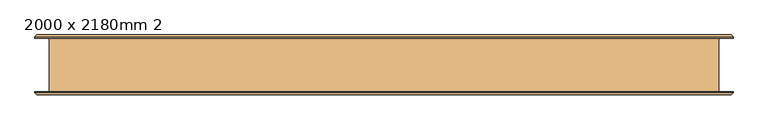
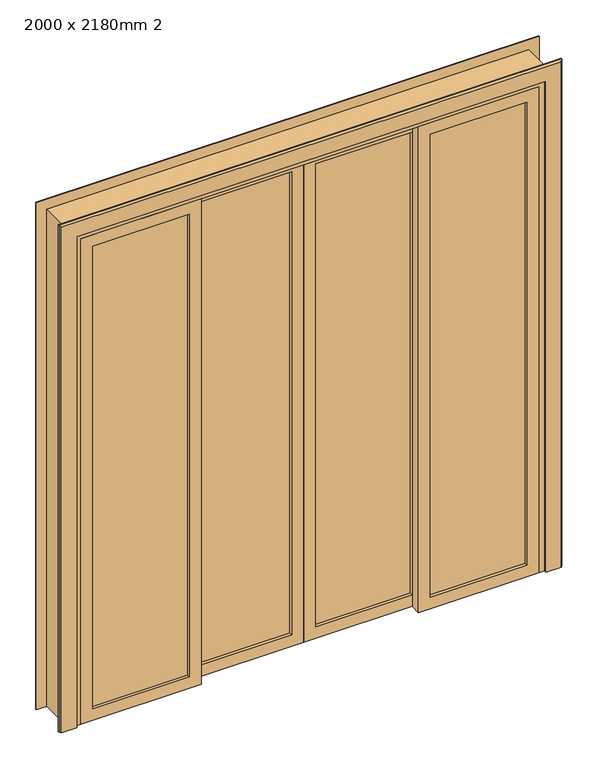
"""IFC4 building model written with IfcOpenShell, lengths in millimetres: door geometry, Porta envidraçada de correr quádrupla com revestimento : 2000 x 2180mm 2."""

from ifc_helpers import new_model, si_unit, point, frame, frame_2d, origin, place, context, project, spatial, polyline, circle_curve, trimmed, segment, composite_curve, outline, extrude, faceted_brep, source, transform, mapped, element, save


def door_2000_x_2180mm_2_8f6b41c2(model_context):
    return source(origin(), model_context, "Body", "SolidModel", [
        extrude(outline(composite_curve([segment(trimmed(circle_curve(frame_2d((990.0, 15.0)), 10.0), [point((1000.0, 15.0))], [point((990.0, 5.0))], False, "CARTESIAN"), True, "CONTINUOUS"), segment(polyline([(990.0, 5.0), (810.0, 5.0)]), True, "CONTINUOUS"), segment(trimmed(circle_curve(frame_2d((810.0, 15.0)), 10.0), [point((810.0, 5.0))], [point((800.0, 15.0))], False, "CARTESIAN"), True, "CONTINUOUS"), segment(polyline([(800.0, 15.0), (800.0, 35.0)]), True, "CONTINUOUS"), segment(trimmed(circle_curve(frame_2d((810.0, 35.0)), 10.0), [point((800.0, 35.0))], [point((810.0, 45.0))], False, "CARTESIAN"), True, "CONTINUOUS"), segment(polyline([(810.0, 45.0), (990.0, 45.0)]), True, "CONTINUOUS"), segment(trimmed(circle_curve(frame_2d((990.0, 35.0)), 10.0), [point((990.0, 45.0))], [point((1000.0, 35.0))], False, "CARTESIAN"), True, "CONTINUOUS"), segment(polyline([(1000.0, 35.0), (1000.0, 15.0)]), True, "CONTINUOUS")], self_intersect=False), holes=[composite_curve([segment(trimmed(circle_curve(frame_2d((985.0, 25.0)), 5.0), [point((985.0, 20.0))], [point((985.0, 30.0))], True, "CARTESIAN"), True, "CONTINUOUS"), segment(trimmed(circle_curve(frame_2d((985.0, 25.0)), 5.0), [point((985.0, 30.0))], [point((985.0, 20.0))], True, "CARTESIAN"), True, "CONTINUOUS")], self_intersect=False), composite_curve([segment(trimmed(circle_curve(frame_2d((815.0, 25.0)), 5.0), [point((815.0, 20.0))], [point((815.0, 30.0))], True, "CARTESIAN"), True, "CONTINUOUS"), segment(trimmed(circle_curve(frame_2d((815.0, 25.0)), 5.0), [point((815.0, 30.0))], [point((815.0, 20.0))], True, "CARTESIAN"), True, "CONTINUOUS")], self_intersect=False), composite_curve([segment(polyline([(960.0, 15.0), (960.0, 35.0)]), True, "CONTINUOUS"), segment(trimmed(circle_curve(frame_2d((955.0, 35.0)), 5.0), [point((960.0, 35.0))], [point((955.0, 40.0))], True, "CARTESIAN"), True, "CONTINUOUS"), segment(polyline([(955.0, 40.0), (845.0, 40.0)]), True, "CONTINUOUS"), segment(trimmed(circle_curve(frame_2d((845.0, 35.0)), 5.0), [point((845.0, 40.0))], [point((840.0, 35.0))], True, "CARTESIAN"), True, "CONTINUOUS"), segment(polyline([(840.0, 35.0), (840.0, 15.0)]), True, "CONTINUOUS"), segment(trimmed(circle_curve(frame_2d((845.0, 15.0)), 5.0), [point((840.0, 15.0))], [point((845.0, 10.0))], True, "CARTESIAN"), True, "CONTINUOUS"), segment(polyline([(845.0, 10.0), (955.0, 10.0)]), True, "CONTINUOUS"), segment(trimmed(circle_curve(frame_2d((955.0, 15.0)), 5.0), [point((955.0, 10.0))], [point((960.0, 15.0))], True, "CARTESIAN"), True, "CONTINUOUS")], self_intersect=False)]), frame((0.0, 5.4, 0.0), z_axis=(0.0, 1.0, 0.0), x_axis=(0.0, 0.0, 1.0)), (0.0, 0.0, 1.0), 3.0),
        extrude(outline(composite_curve([segment(trimmed(circle_curve(frame_2d((990.0, -35.0)), 10.0), [point((1000.0, -35.0))], [point((990.0, -45.0))], False, "CARTESIAN"), True, "CONTINUOUS"), segment(polyline([(990.0, -45.0), (810.0, -45.0)]), True, "CONTINUOUS"), segment(trimmed(circle_curve(frame_2d((810.0, -35.0)), 10.0), [point((810.0, -45.0))], [point((800.0, -35.0))], False, "CARTESIAN"), True, "CONTINUOUS"), segment(polyline([(800.0, -35.0), (800.0, -15.0)]), True, "CONTINUOUS"), segment(trimmed(circle_curve(frame_2d((810.0, -15.0)), 10.0), [point((800.0, -15.0))], [point((810.0, -5.0))], False, "CARTESIAN"), True, "CONTINUOUS"), segment(polyline([(810.0, -5.0), (990.0, -5.0)]), True, "CONTINUOUS"), segment(trimmed(circle_curve(frame_2d((990.0, -15.0)), 10.0), [point((990.0, -5.0))], [point((1000.0, -15.0))], False, "CARTESIAN"), True, "CONTINUOUS"), segment(polyline([(1000.0, -15.0), (1000.0, -35.0)]), True, "CONTINUOUS")], self_intersect=False), holes=[composite_curve([segment(trimmed(circle_curve(frame_2d((985.0, -25.0)), 5.0), [point((985.0, -30.0))], [point((985.0, -20.0))], True, "CARTESIAN"), True, "CONTINUOUS"), segment(trimmed(circle_curve(frame_2d((985.0, -25.0)), 5.0), [point((985.0, -20.0))], [point((985.0, -30.0))], True, "CARTESIAN"), True, "CONTINUOUS")], self_intersect=False), composite_curve([segment(trimmed(circle_curve(frame_2d((815.0, -25.0)), 5.0), [point((815.0, -30.0))], [point((815.0, -20.0))], True, "CARTESIAN"), True, "CONTINUOUS"), segment(trimmed(circle_curve(frame_2d((815.0, -25.0)), 5.0), [point((815.0, -20.0))], [point((815.0, -30.0))], True, "CARTESIAN"), True, "CONTINUOUS")], self_intersect=False), composite_curve([segment(polyline([(960.0, -35.0), (960.0, -15.0)]), True, "CONTINUOUS"), segment(trimmed(circle_curve(frame_2d((955.0, -15.0)), 5.0), [point((960.0, -15.0))], [point((955.0, -10.0))], True, "CARTESIAN"), True, "CONTINUOUS"), segment(polyline([(955.0, -10.0), (845.0, -10.0)]), True, "CONTINUOUS"), segment(trimmed(circle_curve(frame_2d((845.0, -15.0)), 5.0), [point((845.0, -10.0))], [point((840.0, -15.0))], True, "CARTESIAN"), True, "CONTINUOUS"), segment(polyline([(840.0, -15.0), (840.0, -35.0)]), True, "CONTINUOUS"), segment(trimmed(circle_curve(frame_2d((845.0, -35.0)), 5.0), [point((840.0, -35.0))], [point((845.0, -40.0))], True, "CARTESIAN"), True, "CONTINUOUS"), segment(polyline([(845.0, -40.0), (955.0, -40.0)]), True, "CONTINUOUS"), segment(trimmed(circle_curve(frame_2d((955.0, -35.0)), 5.0), [point((955.0, -40.0))], [point((960.0, -35.0))], True, "CARTESIAN"), True, "CONTINUOUS")], self_intersect=False)]), frame((0.0, 5.4, 0.0), z_axis=(0.0, 1.0, 0.0), x_axis=(0.0, 0.0, 1.0)), (0.0, 0.0, 1.0), 3.0),
        extrude(outline(polyline([(2130.0, -500.0), (0.0, -500.0), (0.0, 0.0), (2130.0, 0.0), (2130.0, -500.0)]), holes=[polyline([(2080.0, -50.0), (50.0, -50.0), (50.0, -450.0), (2080.0, -450.0), (2080.0, -50.0)])]), frame((0.0, -34.6, 0.0), z_axis=(0.0, 1.0, 0.0), x_axis=(0.0, 0.0, 1.0)), (0.0, 0.0, 1.0), 40.0),
        extrude(outline(polyline([(2130.0, 450.0), (0.0, 450.0), (0.0, 950.0), (2130.0, 950.0), (2130.0, 450.0)]), holes=[polyline([(2080.0, 900.0), (50.0, 900.0), (50.0, 500.0), (2080.0, 500.0), (2080.0, 900.0)])]), frame((0.0, -79.6, 0.0), z_axis=(0.0, 1.0, 0.0), x_axis=(0.0, 0.0, 1.0)), (0.0, 0.0, 1.0), 40.0),
        extrude(outline(polyline([(2130.0, 0.0), (0.0, 0.0), (0.0, 500.0), (2130.0, 500.0), (2130.0, 0.0)]), holes=[polyline([(2080.0, 450.0), (50.0, 450.0), (50.0, 50.0), (2080.0, 50.0), (2080.0, 450.0)])]), frame((0.0, -34.6, 0.0), z_axis=(0.0, 1.0, 0.0), x_axis=(0.0, 0.0, 1.0)), (0.0, 0.0, 1.0), 40.0),
        extrude(outline(polyline([(2130.0, -950.0), (0.0, -950.0), (0.0, -450.0), (2130.0, -450.0), (2130.0, -950.0)]), holes=[polyline([(2080.0, -500.0), (50.0, -500.0), (50.0, -900.0), (2080.0, -900.0), (2080.0, -500.0)])]), frame((0.0, -79.6, 0.0), z_axis=(0.0, 1.0, 0.0), x_axis=(0.0, 0.0, 1.0)), (0.0, 0.0, 1.0), 40.0),
        extrude(outline(polyline([(0.0, 950.0), (0.0, 1000.0), (2180.0, 1000.0), (2180.0, -1000.0), (0.0, -1000.0), (0.0, -950.0), (2130.0, -950.0), (2130.0, 950.0), (0.0, 950.0)])), frame((0.0, -79.6, 0.0), z_axis=(0.0, 1.0, 0.0), x_axis=(0.0, 0.0, 1.0)), (0.0, 0.0, 1.0), 159.2),
        extrude(outline(polyline([(450.0, -7.6), (450.0, -21.6), (50.0, -21.6), (50.0, -7.6), (450.0, -7.6)])), frame((0.0, 0.0, 50.0), z_axis=(0.0, 0.0, 1.0), x_axis=(1.0, 0.0, 0.0)), (0.0, 0.0, 1.0), 2030.0),
        extrude(outline(polyline([(900.0, -52.6), (900.0, -66.6), (500.0, -66.6), (500.0, -52.6), (900.0, -52.6)])), frame((0.0, 0.0, 50.0), z_axis=(0.0, 0.0, 1.0), x_axis=(1.0, 0.0, 0.0)), (0.0, 0.0, 1.0), 2030.0),
        extrude(outline(polyline([(-500.0, -52.6), (-500.0, -66.6), (-900.0, -66.6), (-900.0, -52.6), (-500.0, -52.6)])), frame((0.0, 0.0, 50.0), z_axis=(0.0, 0.0, 1.0), x_axis=(1.0, 0.0, 0.0)), (0.0, 0.0, 1.0), 2030.0),
        extrude(outline(polyline([(-50.0, -7.6), (-50.0, -21.6), (-450.0, -21.6), (-450.0, -7.6), (-50.0, -7.6)])), frame((0.0, 0.0, 50.0), z_axis=(0.0, 0.0, 1.0), x_axis=(1.0, 0.0, 0.0)), (0.0, 0.0, 1.0), 2030.0),
        extrude(outline(polyline([(-500.0, -52.6), (-500.0, -66.6), (-900.0, -66.6), (-900.0, -52.6), (-500.0, -52.6)])), frame((0.0, 0.0, 50.0), z_axis=(0.0, 0.0, 1.0), x_axis=(1.0, 0.0, 0.0)), (0.0, 0.0, 1.0), 2030.0),
        extrude(outline(polyline([(-50.0, -7.6), (-50.0, -21.6), (-450.0, -21.6), (-450.0, -7.6), (-50.0, -7.6)])), frame((0.0, 0.0, 50.0), z_axis=(0.0, 0.0, 1.0), x_axis=(1.0, 0.0, 0.0)), (0.0, 0.0, 1.0), 2030.0),
        extrude(outline(polyline([(500.0, -52.6), (900.0, -52.6), (900.0, -66.6), (500.0, -66.6), (500.0, -52.6)])), frame((0.0, 0.0, 50.0), z_axis=(0.0, 0.0, 1.0), x_axis=(1.0, 0.0, 0.0)), (0.0, 0.0, 1.0), 2030.0),
        extrude(outline(polyline([(50.0, -7.6), (450.0, -7.6), (450.0, -21.6), (50.0, -21.6), (50.0, -7.6)])), frame((0.0, 0.0, 50.0), z_axis=(0.0, 0.0, 1.0), x_axis=(1.0, 0.0, 0.0)), (0.0, 0.0, 1.0), 2030.0),
        faceted_brep([(1043.0, 83.6, 0.0), (1043.0, 79.6, 0.0), (973.0, 79.6, 0.0), (973.0, 89.6, 0.0), (1037.0, 89.6, 0.0), (1043.0, 83.6, 2223.0), (1043.0, 79.6, 2223.0), (-1043.0, 79.6, 2223.0), (-1043.0, 79.6, 0.0), (-973.0, 79.6, 0.0), (-973.0, 79.6, 2153.0), (973.0, 79.6, 2153.0), (973.0, 89.6, 2153.0), (-973.0, 89.6, 2153.0), (-973.0, 89.6, 0.0), (-1037.0, 89.6, 0.0), (-1037.0, 89.6, 2217.0), (1037.0, 89.6, 2217.0), (-1043.0, 83.6, 0.0), (-1043.0, 83.6, 2223.0)], [[[0, 1, 2, 3, 4]], [[1, 0, 5, 6]], [[2, 1, 6, 7, 8, 9, 10, 11]], [[3, 2, 11, 12]], [[4, 3, 12, 13, 14, 15, 16, 17]], [[0, 4, 17, 5]], [[13, 10, 9, 14]], [[18, 15, 14, 9, 8]], [[19, 16, 15, 18]], [[7, 19, 18, 8]], [[5, 17, 16, 19]], [[12, 11, 10, 13]], [[6, 5, 19, 7]]]),
        faceted_brep([(1043.0, -83.6, 0.0), (1037.0, -89.6, 0.0), (973.0, -89.6, 0.0), (973.0, -79.6, 0.0), (1043.0, -79.6, 0.0), (1043.0, -83.6, 2223.0), (1037.0, -89.6, 2217.0), (-1037.0, -89.6, 2217.0), (-1037.0, -89.6, 0.0), (-973.0, -89.6, 0.0), (-973.0, -89.6, 2153.0), (973.0, -89.6, 2153.0), (973.0, -79.6, 2153.0), (-973.0, -79.6, 2153.0), (-973.0, -79.6, 0.0), (-1043.0, -79.6, 0.0), (-1043.0, -79.6, 2223.0), (1043.0, -79.6, 2223.0), (-1043.0, -83.6, 2223.0), (-1043.0, -83.6, 0.0)], [[[0, 1, 2, 3, 4]], [[1, 0, 5, 6]], [[2, 1, 6, 7, 8, 9, 10, 11]], [[3, 2, 11, 12]], [[4, 3, 12, 13, 14, 15, 16, 17]], [[0, 4, 17, 5]], [[7, 18, 19, 8]], [[19, 15, 14, 9, 8]], [[13, 10, 9, 14]], [[18, 16, 15, 19]], [[6, 5, 18, 7]], [[12, 11, 10, 13]], [[5, 17, 16, 18]]]),
    ])


if __name__ == "__main__":
    model = new_model("IFC4")
    model_context = context("Model", 3, world=origin())
    ifc_project = project(units=[si_unit("LENGTHUNIT", "METRE", prefix="MILLI")], contexts=[model_context])
    site = spatial("IfcSite", under=ifc_project)
    building = spatial("IfcBuilding", under=site)
    placement = place(None, origin())
    door_2000_x_2180mm_2_shape = door_2000_x_2180mm_2_8f6b41c2(model_context)
    element("IfcDoor", 1, ObjectType="Porta envidraçada de correr quádrupla com revestimento : 2000 x 2180mm 2", at=placement, inside=building, context=model_context, shape_type="MappedRepresentation", body=[
        mapped(door_2000_x_2180mm_2_shape, transform((0.0, 0.0, 0.0), x_axis=(1.0, 0.0, 0.0), y_axis=(0.0, 1.0, 0.0), z_axis=(0.0, 0.0, 1.0))),
    ])
    save(model, "model.ifc")

# Revit data of these elements
# Type "Porta envidraçada de correr quádrupla com revestimento : 2000 x 2180mm 2"
#   Type Mark = "P42"
#   Construction Type Id = "GSP4R"
#   Analytic Construction = "Vidraça única Pilkington 1/8 pol"
#   Visual Light Transmittance = 0.9
#   Largura da apara = 0.07 m
#   Espessura da apara = 0.01 m
#   Solar Heat Gain Coefficient = 0.78
#   Rough Width = 2.00 m
#   Rough Height = 2.18 m
#   Largura da moldura do painel = 0.05 m
#   Espessura da moldura do painel = 0.04 m
#   Heat Transfer Coefficient (U) = 3.6886 W/(m²·K)
#   Largura da maçaneta = 0.04 m
#   Altura do puxador = 0.20 m
#   Largura da estrutura = 0.05 m
#   Height = 2.18 m
#   Width = 2.00 m
#   Function = 1
#   Material da apara = none
#   Material do puxador = none
#   Vidro = Vidro
#   Material da estrutura = none
#   Thickness = 0
#   Wall Closure = (empty or 0)
# Element 1 (IfcDoor, "Porta envidraçada de correr quádrupla com revestimento : 2000 x 2180mm 2")
#   Materials on its faces: "Vidro"
# Materials
#   "Vidro": class "Vidro", colour RGB 0 128 192, transparency 0.9, Description = "Vidro de sílica", Cost = 0
